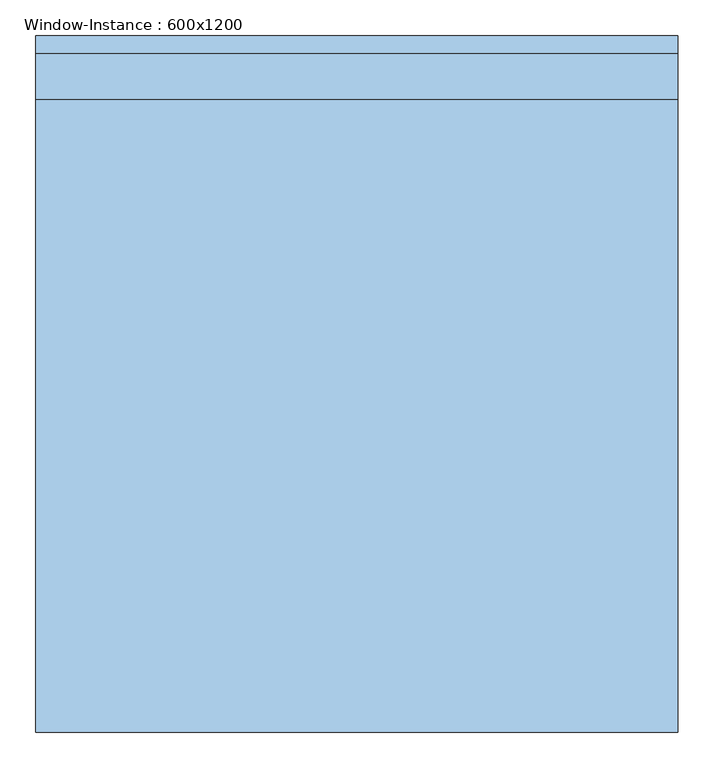
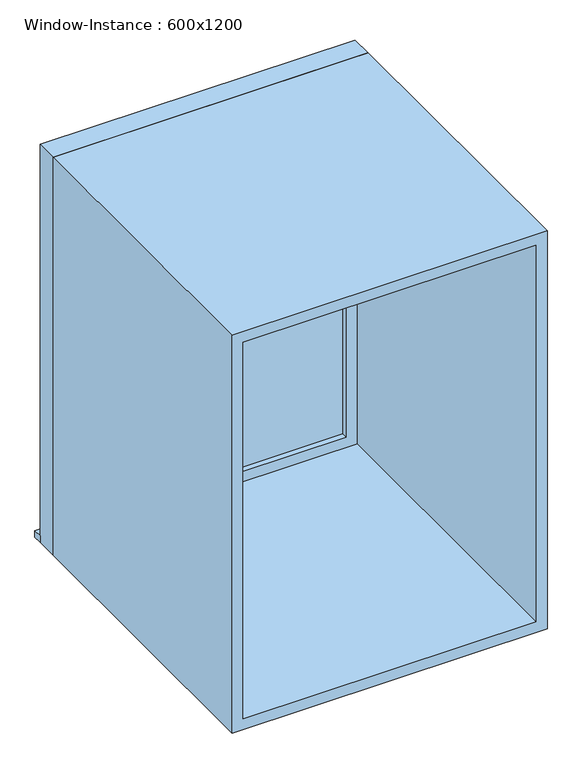
"""IFC4 building model written with IfcOpenShell, lengths in millimetres: window geometry, Window-Instance : 600x1200."""

from ifc_helpers import new_model, si_unit, frame, origin, place, context, project, spatial, polyline, outline, extrude, source, transform, mapped, element, save


def window_instance_600x1200_24f0490b(model_context):
    return source(origin(), model_context, "Body", "SweptSolid", [
        extrude(outline(polyline([(-488.1, 500.4), (411.9, 500.4), (411.9, 475.0), (-488.1, 475.0), (-488.1, 500.4)])), frame((0.0, 0.0, 900.0), z_axis=(0.0, 0.0, 1.0), x_axis=(1.0, 0.0, 0.0)), (0.0, 0.0, 1.0), 19.05),
        extrude(outline(polyline([(348.4, 426.425), (-424.6, 426.425), (-424.6, 439.125), (348.4, 439.125), (348.4, 426.425)])), frame((0.0, 0.0, 963.5), z_axis=(0.0, 0.0, 1.0), x_axis=(1.0, 0.0, 0.0)), (0.0, 0.0, 1.0), 1073.0),
        extrude(outline(polyline([(2080.95, -469.05), (919.05, -469.05), (919.05, 392.85), (2080.95, 392.85), (2080.95, -469.05)]), holes=[polyline([(2036.5, -424.6), (2036.5, 348.4), (963.5, 348.4), (963.5, -424.6), (2036.5, -424.6)])]), frame((0.0, 410.55, 0.0), z_axis=(0.0, 1.0, 0.0), x_axis=(0.0, 0.0, 1.0)), (0.0, 0.0, 1.0), 44.45),
        extrude(outline(polyline([(2100.0, -488.1), (900.0, -488.1), (900.0, 411.9), (2100.0, 411.9), (2100.0, -488.1)]), holes=[polyline([(2068.25, -456.35), (2068.25, 380.15), (931.75, 380.15), (931.75, -456.35), (2068.25, -456.35)])]), frame((0.0, -475.0, 0.0), z_axis=(0.0, 1.0, 0.0), x_axis=(0.0, 0.0, 1.0)), (0.0, 0.0, 1.0), 885.55),
        extrude(outline(polyline([(2100.0, 411.9), (2100.0, -488.1), (900.0, -488.1), (900.0, 411.9), (2100.0, 411.9)]), holes=[polyline([(2080.95, 392.85), (919.05, 392.85), (919.05, -469.05), (2080.95, -469.05), (2080.95, 392.85)])]), frame((0.0, 410.55, 0.0), z_axis=(0.0, 1.0, 0.0), x_axis=(0.0, 0.0, 1.0)), (0.0, 0.0, 1.0), 64.45),
    ])


if __name__ == "__main__":
    model = new_model("IFC4")
    model_context = context("Model", 3, world=origin())
    ifc_project = project(units=[si_unit("LENGTHUNIT", "METRE", prefix="MILLI")], contexts=[model_context])
    site = spatial("IfcSite", under=ifc_project)
    building = spatial("IfcBuilding", under=site)
    placement = place(None, origin())
    window_instance_600x1200_shape = window_instance_600x1200_24f0490b(model_context)
    element("IfcWindow", 1, ObjectType="Window-Instance : 600x1200", at=placement, inside=building, context=model_context, shape_type="MappedRepresentation", body=[
        mapped(window_instance_600x1200_shape, transform((0.0, 0.0, 0.0), x_axis=(1.0, 0.0, 0.0), y_axis=(0.0, 1.0, 0.0), z_axis=(0.0, 0.0, 1.0))),
    ])
    save(model, "model.ifc")

# Revit data of these elements
# Type "Window-Instance : 600x1200"
#   Type Mark = "7"
#   Construction Type Id = "GSP4R"
#   Assembly Code = "B2020100"
#   Analytic Construction = "1/8 in Pilkington single glazing"
#   Visual Light Transmittance = 0.9
#   Thermal Resistance (R) = 0.149095 (m²·K)/W
#   Solar Heat Gain Coefficient = 0.86
#   Heat Transfer Coefficient (U) = 6.70716 W/(m²·K)
#   Height [instance default] = 1200 mm
#   Default Sill Height = 900 mm
#   Width [instance default] = 600 mm
#   Window Inset = 20 mm
#   Glass Pane Material = WW-EC-GL-Storefront
#   Sash Material = WW-EC-RGB-White
#   Wall Closure = (empty or 0)
# Element 1 (IfcWindow, "Window-Instance : 600x1200")
#   Width = 900 mm
#   Materials on its faces: "WW-EC-RGB-White", "WW-EC-GL-Storefront"
# Materials
#   "WW-EC-GL-Storefront": class "Glass", colour RGB 236 240 239, transparency 0.85, Description = "Storefront Glass", Cost = 0
#   "WW-EC-RGB-White": class "Generic", colour RGB 255 255 255, transparency 0, Comments = "If region requests off-white, swith asset color to RGB 231-228-220", Description = "Generic Color", Cost = 0
